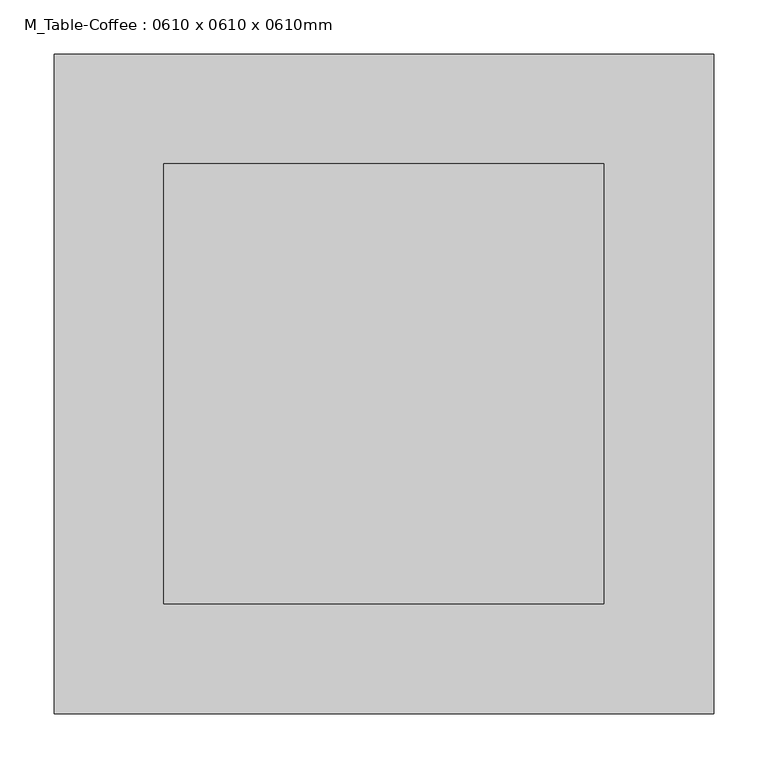
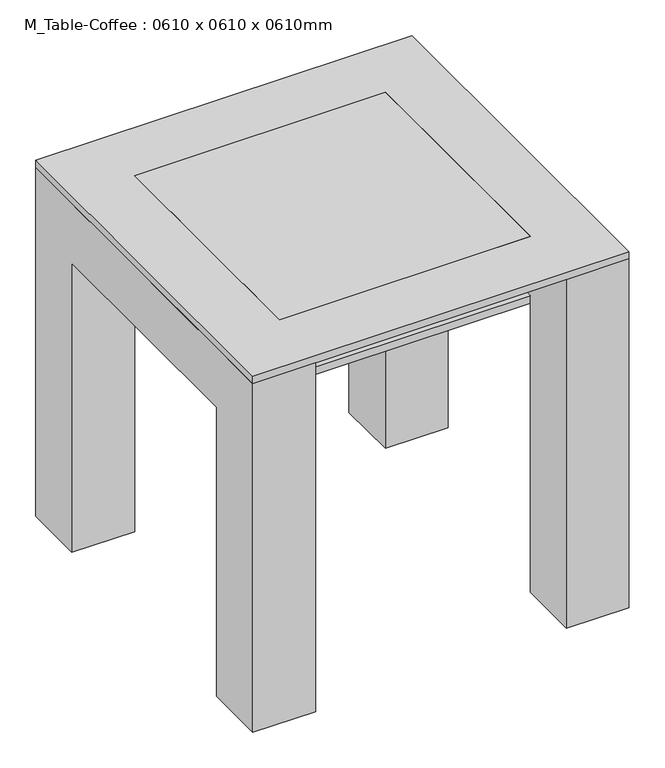
"""IFC4 building model written with IfcOpenShell, lengths in millimetres: furniture geometry, M_Table-Coffee : 0610 x 0610 x 0610mm."""

import ifcopenshell
import ifcopenshell.guid

model = None  # the IFC model being written
_history = None  # IfcOwnerHistory: only IFC2X3 demands one
_inside = {}  # id of a spatial element -> (the spatial element, [elements in it])
_under = {}  # id of a project, library or spatial element -> (it, [spatial elements below it])
_declared = {}  # id of a project -> (the project, [libraries it declares])
_typed = {}  # id of a type object -> (the type object, [elements of that type])
_made_of = {}  # id of a material, layer set ... -> (it, [elements and type objects made of it])


def new_model(schema):
    """Start an empty IFC model of exactly this schema.

    Asked for "IFC4X3", IfcOpenShell would pick the latest addendum, in which some entities
    have other attributes; the version numbers below select the first issue.
    IFC2X3 requires an IfcOwnerHistory on every rooted entity: one is made here for all.
    """
    global model, _history
    if schema == "IFC4X3":
        model = ifcopenshell.file(schema_version=(4, 3, 0, 0))
    else:
        model = ifcopenshell.file(schema=schema)
    _inside.clear()
    _under.clear()
    _declared.clear()
    _typed.clear()
    _made_of.clear()
    _history = None
    if model.schema == "IFC2X3":
        org = make("IfcOrganization", Name="unknown")
        user = make(
            "IfcPersonAndOrganization",
            ThePerson=make("IfcPerson", FamilyName="unknown"),
            TheOrganization=org,
        )
        app = make(
            "IfcApplication",
            ApplicationDeveloper=org,
            Version="unknown",
            ApplicationFullName="unknown",
            ApplicationIdentifier="unknown",
        )
        _history = make(
            "IfcOwnerHistory",
            OwningUser=user,
            OwningApplication=app,
            ChangeAction="ADDED",
            CreationDate=0,
        )
    return model


def make(cls, **values):
    """One entity of the class cls with the attributes given. An attribute that is None is left unset."""
    return model.create_entity(
        cls, **{name: value for name, value in values.items() if value is not None}
    )


def rooted(cls, **values):
    """An entity with a GlobalId (a new one), such as an element, a storey or a relation."""
    return make(cls, GlobalId=ifcopenshell.guid.new(), OwnerHistory=_history, **values)


def si_unit(unit_type, name, prefix=None):
    """IfcSIUnit, for example si_unit("LENGTHUNIT", "METRE", prefix="MILLI")."""
    return make("IfcSIUnit", UnitType=unit_type, Prefix=prefix, Name=name)


def assignment(units):
    """IfcUnitAssignment: the units of a project."""
    return None if units is None else make("IfcUnitAssignment", Units=units)


def point(xyz):
    """IfcCartesianPoint."""
    return None if xyz is None else make("IfcCartesianPoint", Coordinates=xyz)


def direction(xyz):
    """IfcDirection."""
    return None if xyz is None else make("IfcDirection", DirectionRatios=xyz)


def frame(location, z_axis=None, x_axis=None):
    """IfcAxis2Placement3D, a coordinate frame: its origin and axes. An axis left out is left unset."""
    return make(
        "IfcAxis2Placement3D",
        Location=point(location),
        Axis=direction(z_axis),
        RefDirection=direction(x_axis),
    )


def origin():
    """The frame at (0, 0, 0) with its axes left unset."""
    return frame((0.0, 0.0, 0.0))


def place(relative_to, where):
    """IfcLocalPlacement: puts the frame where relative to a parent placement (None: the world)."""
    return make(
        "IfcLocalPlacement", PlacementRelTo=relative_to, RelativePlacement=where
    )


def context(
    kind, dimensions, precision=None, world=None, true_north=None, identifier=None
):
    """IfcGeometricRepresentationContext, for example the 3D "Model" context."""
    return make(
        "IfcGeometricRepresentationContext",
        ContextIdentifier=identifier,
        ContextType=kind,
        CoordinateSpaceDimension=dimensions,
        Precision=precision,
        WorldCoordinateSystem=world,
        TrueNorth=true_north,
    )


def project(units=None, contexts=None):
    """IfcProject with its units and contexts."""
    return rooted(
        "IfcProject",
        Name="project",
        RepresentationContexts=contexts,
        UnitsInContext=assignment(units),
    )


def spatial(cls, under=None, at=None, **own):
    """A site, building, storey or space (cls), placed at a placement, below another one or the project."""
    s = rooted(cls, ObjectPlacement=at, **own)
    if under is not None:
        _under.setdefault(under.id(), (under, []))[1].append(s)
    return s


def polyline(points):
    """IfcPolyline through the points."""
    return make("IfcPolyline", Points=[point(p) for p in points])


def outline(outer, holes=None, kind="AREA"):
    """IfcArbitraryClosedProfileDef: a profile drawn as a closed curve; with holes, ...WithVoids."""
    if holes is None:
        return make("IfcArbitraryClosedProfileDef", ProfileType=kind, OuterCurve=outer)
    return make(
        "IfcArbitraryProfileDefWithVoids",
        ProfileType=kind,
        OuterCurve=outer,
        InnerCurves=holes,
    )


def extrude(swept, where, along, depth):
    """IfcExtrudedAreaSolid: the profile swept, set in the frame where, extruded along a direction by depth."""
    return make(
        "IfcExtrudedAreaSolid",
        SweptArea=swept,
        Position=where,
        ExtrudedDirection=direction(along),
        Depth=depth,
    )


def shape(context_of_items, identifier, shape_type, items):
    """IfcShapeRepresentation: the items that make up one representation, for example the "Body"."""
    return make(
        "IfcShapeRepresentation",
        ContextOfItems=context_of_items,
        RepresentationIdentifier=identifier,
        RepresentationType=shape_type,
        Items=items,
    )


def source(mapping_origin, context_of_items, identifier, shape_type, items):
    """IfcRepresentationMap: a shape defined once, which mapped items show again and again."""
    return make(
        "IfcRepresentationMap",
        MappingOrigin=mapping_origin,
        MappedRepresentation=shape(context_of_items, identifier, shape_type, items),
    )


def transform(
    local_origin,
    x_axis=None,
    y_axis=None,
    z_axis=None,
    scale=None,
    scale2=None,
    scale3=None,
    uniform=True,
):
    """IfcCartesianTransformationOperator3D, or its non-uniform kind. x_axis, y_axis, z_axis: its Axis1, 2, 3."""
    if uniform:
        return make(
            "IfcCartesianTransformationOperator3D",
            Axis1=direction(x_axis),
            Axis2=direction(y_axis),
            LocalOrigin=point(local_origin),
            Scale=scale,
            Axis3=direction(z_axis),
        )
    return make(
        "IfcCartesianTransformationOperator3DnonUniform",
        Axis1=direction(x_axis),
        Axis2=direction(y_axis),
        LocalOrigin=point(local_origin),
        Scale=scale,
        Axis3=direction(z_axis),
        Scale2=scale2,
        Scale3=scale3,
    )


def mapped(mapping_source, mapping_target):
    """IfcMappedItem: shows the shape of a source again, moved by a transform."""
    return make(
        "IfcMappedItem", MappingSource=mapping_source, MappingTarget=mapping_target
    )


def made_of(thing, what):
    """Note that an element or type object is made of a material, layer set ...; save() writes the relation."""
    if what is not None:
        _made_of.setdefault(what.id(), (what, []))[1].append(thing)
    return thing


def element(
    cls,
    number,
    at=None,
    inside=None,
    cuts=None,
    type_object=None,
    material=None,
    context=None,
    identifier="Body",
    shape_type=None,
    held_by="IfcProductDefinitionShape",
    body=None,
    shapes=None,
    **own,
):
    """One element of the class cls, such as IfcWall. Its Tag is "e" and its number.

    at: its placement. inside: the storey or other place that contains it. cuts: it is an
    opening in that element (IfcRelVoidsElement). A single representation is given by context,
    identifier, shape_type and body (its items); several are given by shapes. held_by: the class
    of the entity that holds the representations. save() writes the other relations.
    """
    e = rooted(cls, Tag="e%d" % number, ObjectPlacement=at, **own)
    if body is not None:
        shapes = [shape(context, identifier, shape_type, body)]
    if shapes is not None:
        e.Representation = make(held_by, Representations=shapes)
    if inside is not None:
        _inside.setdefault(inside.id(), (inside, []))[1].append(e)
    if cuts is not None:
        rooted(
            "IfcRelVoidsElement", RelatingBuildingElement=cuts, RelatedOpeningElement=e
        )
    if type_object is not None:
        _typed.setdefault(type_object.id(), (type_object, []))[1].append(e)
    return made_of(e, material)


def aggregate(whole, parts):
    """IfcRelAggregates: a whole, such as a stair, and the parts it consists of."""
    return rooted("IfcRelAggregates", RelatingObject=whole, RelatedObjects=parts)


def save(model, path):
    """Write the relations noted so far, then the file.

    IfcRelAggregates (storeys below a building ...), IfcRelContainedInSpatialStructure (elements
    in a storey), IfcRelDefinesByType, IfcRelAssociatesMaterial and IfcRelDeclares: one each for
    every whole, place, type object, material and project.
    """
    for whole, parts in _under.values():
        aggregate(whole, parts)
    for where, things in _inside.values():
        rooted(
            "IfcRelContainedInSpatialStructure",
            RelatedElements=things,
            RelatingStructure=where,
        )
    for kind, things in _typed.values():
        rooted("IfcRelDefinesByType", RelatedObjects=things, RelatingType=kind)
    for what, things in _made_of.values():
        rooted("IfcRelAssociatesMaterial", RelatedObjects=things, RelatingMaterial=what)
    for by, libraries in _declared.values():
        rooted("IfcRelDeclares", RelatingContext=by, RelatedDefinitions=libraries)
    model.write(path)


def m_table_coffee_0610_x_0610_x_0610mm_65ce43c2(model_context):
    return source(origin(), model_context, "Body", "SweptSolid", [
        extrude(outline(polyline([(221.6657667, 298.6110778), (221.6657667, -108.1889222), (-185.1342333, -108.1889222), (-185.1342333, 298.6110778), (221.6657667, 298.6110778)])), frame((0.0, 0.0, 495.7), z_axis=(0.0, 0.0, 1.0), x_axis=(1.0, 0.0, 0.0)), (0.0, 0.0, 1.0), 12.7),
        extrude(outline(polyline([(400.2110778, 0.0), (298.6110778, 0.0), (298.6110778, 495.7), (-108.1889222, 495.7), (-108.1889222, 0.0), (-209.7889222, 0.0), (-209.7889222, 597.3), (400.2110778, 597.3), (400.2110778, 0.0)])), frame((221.6657667, 0.0, 0.0), z_axis=(1.0, 0.0, 0.0), x_axis=(0.0, 1.0, 0.0)), (0.0, 0.0, 1.0), 101.6),
        extrude(outline(polyline([(400.2110778, 597.3), (400.2110778, 0.0), (298.6110778, 0.0), (298.6110778, 495.7), (-108.1889222, 495.7), (-108.1889222, 0.0), (-209.7889222, 0.0), (-209.7889222, 597.3), (400.2110778, 597.3)])), frame((-286.7342333, 0.0, 0.0), z_axis=(1.0, 0.0, 0.0), x_axis=(0.0, 1.0, 0.0)), (0.0, 0.0, 1.0), 101.6),
        extrude(outline(polyline([(221.6657667, 298.6110778), (221.6657667, -108.1889222), (-185.1342333, -108.1889222), (-185.1342333, 298.6110778), (221.6657667, 298.6110778)])), frame((0.0, 0.0, 597.3), z_axis=(0.0, 0.0, 1.0), x_axis=(1.0, 0.0, 0.0)), (0.0, 0.0, 1.0), 12.7),
        extrude(outline(polyline([(323.2657667, 400.2110778), (323.2657667, -209.7889222), (-286.7342333, -209.7889222), (-286.7342333, 400.2110778), (323.2657667, 400.2110778)]), holes=[polyline([(221.6657667, 298.6110778), (-185.1342333, 298.6110778), (-185.1342333, -108.1889222), (221.6657667, -108.1889222), (221.6657667, 298.6110778)])]), frame((0.0, 0.0, 597.3), z_axis=(0.0, 0.0, 1.0), x_axis=(1.0, 0.0, 0.0)), (0.0, 0.0, 1.0), 12.7),
    ])


if __name__ == "__main__":
    model = new_model("IFC4")
    model_context = context("Model", 3, world=origin())
    ifc_project = project(units=[si_unit("LENGTHUNIT", "METRE", prefix="MILLI")], contexts=[model_context])
    site = spatial("IfcSite", under=ifc_project)
    building = spatial("IfcBuilding", under=site)
    placement = place(None, origin())
    m_table_coffee_0610_x_0610_x_0610mm_shape = m_table_coffee_0610_x_0610_x_0610mm_65ce43c2(model_context)
    element("IfcFurniture", 1, ObjectType="M_Table-Coffee : 0610 x 0610 x 0610mm", at=placement, inside=building, context=model_context, shape_type="MappedRepresentation", body=[
        mapped(m_table_coffee_0610_x_0610_x_0610mm_shape, transform((0.0, 0.0, 0.0), x_axis=(1.0, 0.0, 0.0), y_axis=(0.0, 1.0, 0.0), z_axis=(0.0, 0.0, 1.0))),
    ])
    save(model, "model.ifc")

# Revit data of these elements
# Type "M_Table-Coffee : 0610 x 0610 x 0610mm"
#   Manufacturer = "Manufacturer"
#   AccessibilityPerformance = "AccessibilityPerformance"
#   CodePerformance = "CodePerformance"
#   Area = "Area"
#   Color = "Color"
#   Constituents = "Constituents"
#   Features = "Features"
#   Finish = "Finish"
#   Grade = "Grade"
#   Material = "Material"
#   ModelReference = "ModelReference"
#   NominalHeight = "NominalHeight"
#   NominalLength = "NominalLength"
#   NominalWidth = "NominalWidth"
#   ProductionYear = "ProductionYear"
#   Reference = "Reference"
#   Shape = "Shape"
#   Size = "Size"
#   SustainabilityPerformance = "SustainabilityPerformance"
#   WarrantyDescription = "WarrantyDescription"
#   WarrantyDurationLabor = "WarrantyDurationLabor"
#   WarrantyDurationParts = "WarrantyDurationParts"
#   WarrantyGuarantorLabor = "WarrantyGuarantorLabor"
#   WarrantyGuarantorParts = "WarrantyGuarantorParts"
#   ExpectedLife = "ExpectedLife"
#   ReplacementCost = "ReplacementCost"
#   AssetAccountingType = "NONFIXED"
#   ModelLabel = "ModelLabel"
#   Height = 0.610 m
#   Length = 0.610 m
#   Width = 0.610 m
#   Top Material = Metal - Chrome
#   Frame Material = Wood - Teak
# Element 1 (IfcFurniture, "M_Table-Coffee : 0610 x 0610 x 0610mm")
#   Materials on its faces: "Wood - Teak", "Metal - Chrome", "Glass - Clear, Grey"
# Materials
#   "Metal - Chrome": class "Metal", colour RGB 17 17 17, transparency 0
#   "Wood - Teak": class "Wood", colour RGB 145 112 90, transparency 0
#   "Glass - Clear, Grey": class "Glass", colour RGB 252 255 255, transparency 0.64
